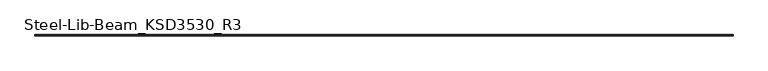
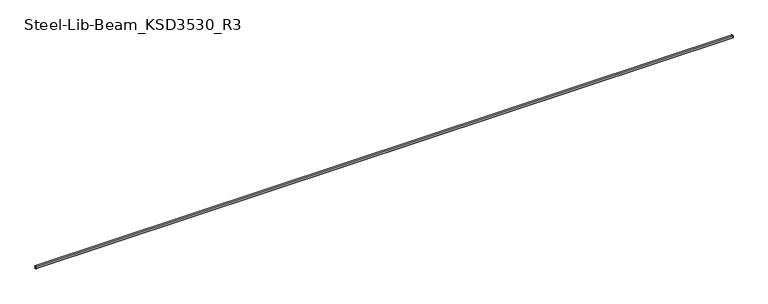
"""IFC4 building model written with IfcOpenShell, lengths in millimetres: beam geometry, Steel-Lib-Beam_KSD3530_R3 : BMS291_C-150×75x20x4.5."""

from ifc_helpers import new_model, si_unit, point, frame, frame_2d, origin, place, context, project, spatial, polyline, circle_curve, trimmed, segment, composite_curve, outline, extrude, source, transform, mapped, element, save


def steel_lib_beam_ksd3530_r3_7619a2e6(model_context):
    return source(origin(), model_context, "Body", "SweptSolid", [
        extrude(outline(composite_curve([segment(polyline([(50.0, 66.0), (50.0, 55.0), (45.5, 55.0), (45.5, 66.0)]), True, "CONTINUOUS"), segment(trimmed(circle_curve(frame_2d((41.0, 66.0)), 4.5), [point((45.5, 66.0))], [point((41.0, 70.5))], True, "CARTESIAN"), True, "CONTINUOUS"), segment(polyline([(41.0, 70.5), (-16.0, 70.5)]), True, "CONTINUOUS"), segment(trimmed(circle_curve(frame_2d((-16.0, 66.0)), 4.5), [point((-16.0, 70.5))], [point((-20.5, 66.0))], True, "CARTESIAN"), True, "CONTINUOUS"), segment(polyline([(-20.5, 66.0), (-20.5, -66.0)]), True, "CONTINUOUS"), segment(trimmed(circle_curve(frame_2d((-16.0, -66.0)), 4.5), [point((-20.5, -66.0))], [point((-16.0, -70.5))], True, "CARTESIAN"), True, "CONTINUOUS"), segment(polyline([(-16.0, -70.5), (41.0, -70.5)]), True, "CONTINUOUS"), segment(trimmed(circle_curve(frame_2d((41.0, -66.0)), 4.5), [point((41.0, -70.5))], [point((45.5, -66.0))], True, "CARTESIAN"), True, "CONTINUOUS"), segment(polyline([(45.5, -66.0), (45.5, -55.0), (50.0, -55.0), (50.0, -66.0)]), True, "CONTINUOUS"), segment(trimmed(circle_curve(frame_2d((41.0, -66.0)), 9.0), [point((50.0, -66.0))], [point((41.0, -75.0))], False, "CARTESIAN"), True, "CONTINUOUS"), segment(polyline([(41.0, -75.0), (-16.0, -75.0)]), True, "CONTINUOUS"), segment(trimmed(circle_curve(frame_2d((-16.0, -66.0)), 9.0), [point((-16.0, -75.0))], [point((-25.0, -66.0))], False, "CARTESIAN"), True, "CONTINUOUS"), segment(polyline([(-25.0, -66.0), (-25.0, 66.0)]), True, "CONTINUOUS"), segment(trimmed(circle_curve(frame_2d((-16.0, 66.0)), 9.0), [point((-25.0, 66.0))], [point((-16.0, 75.0))], False, "CARTESIAN"), True, "CONTINUOUS"), segment(polyline([(-16.0, 75.0), (41.0, 75.0)]), True, "CONTINUOUS"), segment(trimmed(circle_curve(frame_2d((41.0, 66.0)), 9.0), [point((41.0, 75.0))], [point((50.0, 66.0))], False, "CARTESIAN"), True, "CONTINUOUS")], self_intersect=False)), frame((-20487.3, 0.0, 0.0), z_axis=(1.0, 0.0, 0.0), x_axis=(0.0, 1.0, 0.0)), (0.0, 0.0, 1.0), 40924.6),
    ])


if __name__ == "__main__":
    model = new_model("IFC4")
    model_context = context("Model", 3, world=origin())
    ifc_project = project(units=[si_unit("LENGTHUNIT", "METRE", prefix="MILLI")], contexts=[model_context])
    site = spatial("IfcSite", under=ifc_project)
    building = spatial("IfcBuilding", under=site)
    placement = place(None, origin())
    steel_lib_beam_ksd3530_r3_shape = steel_lib_beam_ksd3530_r3_7619a2e6(model_context)
    element("IfcBeam", 1, ObjectType="Steel-Lib-Beam_KSD3530_R3 : BMS291_C-150×75x20x4.5", at=placement, inside=building, context=model_context, shape_type="MappedRepresentation", body=[
        mapped(steel_lib_beam_ksd3530_r3_shape, transform((0.0, 0.0, 0.0), x_axis=(1.0, 0.0, 0.0), y_axis=(0.0, 1.0, 0.0), z_axis=(0.0, 0.0, 1.0))),
    ])
    save(model, "model.ifc")

# Revit data of these elements
# Type "Steel-Lib-Beam_KSD3530_R3 : BMS291_C-150×75x20x4.5"
#   Keynote = "C-150×75x20x4.5"
#   SteelWeight = "Light"
#   x = 0.0250 m
#   t1 = 0.0090 m
#   t = 0.0045 m
#   Surface Area = 0.629834 m²/m
#   Section Area = 13.9688 cm²
#   Mass per Unit Length = 10.9655 kg/m
#   C = 0.0200 m
#   A = 0.0750 m
#   Length [instance default] = 1.5000 m
#   H = 0.1500 m
#   hec_material4 [instance default] = none
#   hec_material3 [instance default] = none
#   hec_material2 [instance default] = none
#   hec_material1 [instance default] = none
#   Structural Material [instance default] = Metal - Steel - Light Gauge
#   Assembly Code = ""
# Element 1 (IfcBeam, "Steel-Lib-Beam_KSD3530_R3 : BMS291_C-150×75x20x4.5")
#   Structural Material = none
# Materials
#   "Metal - Steel - Light Gauge": class "Metal", colour RGB 247 247 247, transparency 0
